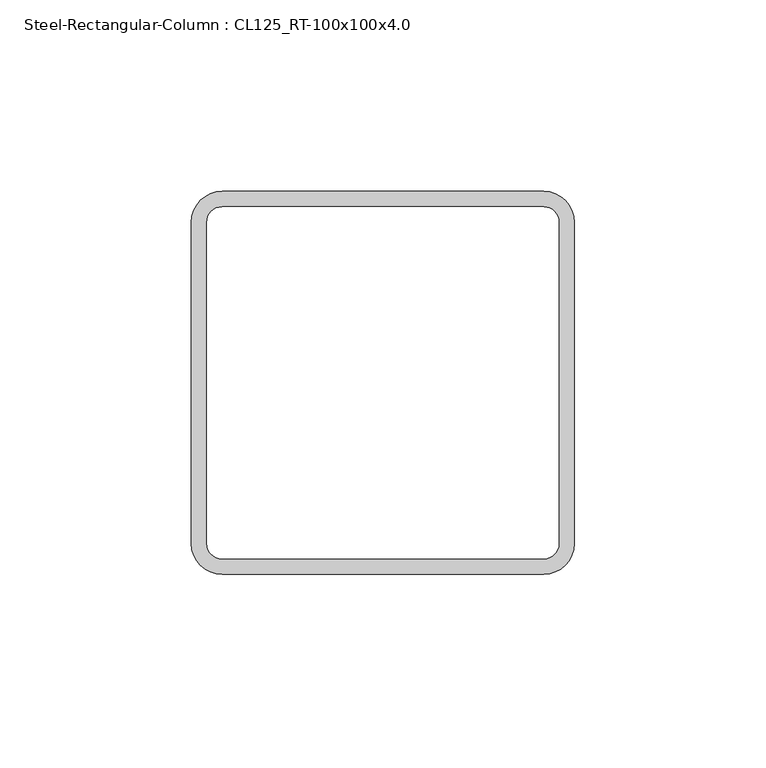
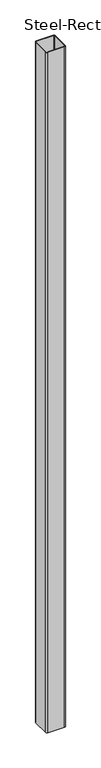
"""IFC4 building model written with IfcOpenShell, lengths in millimetres: column geometry, Steel-Rectangular-Column : CL125_RT-100x100x4.0."""

import ifcopenshell
import ifcopenshell.guid

model = None  # the IFC model being written
_history = None  # IfcOwnerHistory: only IFC2X3 demands one
_inside = {}  # id of a spatial element -> (the spatial element, [elements in it])
_under = {}  # id of a project, library or spatial element -> (it, [spatial elements below it])
_declared = {}  # id of a project -> (the project, [libraries it declares])
_typed = {}  # id of a type object -> (the type object, [elements of that type])
_made_of = {}  # id of a material, layer set ... -> (it, [elements and type objects made of it])


def new_model(schema):
    """Start an empty IFC model of exactly this schema.

    Asked for "IFC4X3", IfcOpenShell would pick the latest addendum, in which some entities
    have other attributes; the version numbers below select the first issue.
    IFC2X3 requires an IfcOwnerHistory on every rooted entity: one is made here for all.
    """
    global model, _history
    if schema == "IFC4X3":
        model = ifcopenshell.file(schema_version=(4, 3, 0, 0))
    else:
        model = ifcopenshell.file(schema=schema)
    _inside.clear()
    _under.clear()
    _declared.clear()
    _typed.clear()
    _made_of.clear()
    _history = None
    if model.schema == "IFC2X3":
        org = make("IfcOrganization", Name="unknown")
        user = make(
            "IfcPersonAndOrganization",
            ThePerson=make("IfcPerson", FamilyName="unknown"),
            TheOrganization=org,
        )
        app = make(
            "IfcApplication",
            ApplicationDeveloper=org,
            Version="unknown",
            ApplicationFullName="unknown",
            ApplicationIdentifier="unknown",
        )
        _history = make(
            "IfcOwnerHistory",
            OwningUser=user,
            OwningApplication=app,
            ChangeAction="ADDED",
            CreationDate=0,
        )
    return model


def make(cls, **values):
    """One entity of the class cls with the attributes given. An attribute that is None is left unset."""
    return model.create_entity(
        cls, **{name: value for name, value in values.items() if value is not None}
    )


def rooted(cls, **values):
    """An entity with a GlobalId (a new one), such as an element, a storey or a relation."""
    return make(cls, GlobalId=ifcopenshell.guid.new(), OwnerHistory=_history, **values)


def si_unit(unit_type, name, prefix=None):
    """IfcSIUnit, for example si_unit("LENGTHUNIT", "METRE", prefix="MILLI")."""
    return make("IfcSIUnit", UnitType=unit_type, Prefix=prefix, Name=name)


def assignment(units):
    """IfcUnitAssignment: the units of a project."""
    return None if units is None else make("IfcUnitAssignment", Units=units)


def point(xyz):
    """IfcCartesianPoint."""
    return None if xyz is None else make("IfcCartesianPoint", Coordinates=xyz)


def direction(xyz):
    """IfcDirection."""
    return None if xyz is None else make("IfcDirection", DirectionRatios=xyz)


def frame(location, z_axis=None, x_axis=None):
    """IfcAxis2Placement3D, a coordinate frame: its origin and axes. An axis left out is left unset."""
    return make(
        "IfcAxis2Placement3D",
        Location=point(location),
        Axis=direction(z_axis),
        RefDirection=direction(x_axis),
    )


def frame_2d(location, x_axis=None):
    """IfcAxis2Placement2D, a coordinate frame in the plane: its origin and x axis."""
    return make(
        "IfcAxis2Placement2D", Location=point(location), RefDirection=direction(x_axis)
    )


def origin():
    """The frame at (0, 0, 0) with its axes left unset."""
    return frame((0.0, 0.0, 0.0))


def place(relative_to, where):
    """IfcLocalPlacement: puts the frame where relative to a parent placement (None: the world)."""
    return make(
        "IfcLocalPlacement", PlacementRelTo=relative_to, RelativePlacement=where
    )


def context(
    kind, dimensions, precision=None, world=None, true_north=None, identifier=None
):
    """IfcGeometricRepresentationContext, for example the 3D "Model" context."""
    return make(
        "IfcGeometricRepresentationContext",
        ContextIdentifier=identifier,
        ContextType=kind,
        CoordinateSpaceDimension=dimensions,
        Precision=precision,
        WorldCoordinateSystem=world,
        TrueNorth=true_north,
    )


def project(units=None, contexts=None):
    """IfcProject with its units and contexts."""
    return rooted(
        "IfcProject",
        Name="project",
        RepresentationContexts=contexts,
        UnitsInContext=assignment(units),
    )


def spatial(cls, under=None, at=None, **own):
    """A site, building, storey or space (cls), placed at a placement, below another one or the project."""
    s = rooted(cls, ObjectPlacement=at, **own)
    if under is not None:
        _under.setdefault(under.id(), (under, []))[1].append(s)
    return s


def polyline(points):
    """IfcPolyline through the points."""
    return make("IfcPolyline", Points=[point(p) for p in points])


def circle_curve(where, radius):
    """IfcCircle in the frame where."""
    return make("IfcCircle", Position=where, Radius=radius)


def trimmed(basis, trim1, trim2, sense, master):
    """IfcTrimmedCurve: the piece of a basis curve between two trims."""
    return make(
        "IfcTrimmedCurve",
        BasisCurve=basis,
        Trim1=trim1,
        Trim2=trim2,
        SenseAgreement=sense,
        MasterRepresentation=master,
    )


def segment(curve, same_sense, transition):
    """IfcCompositeCurveSegment."""
    return make(
        "IfcCompositeCurveSegment",
        Transition=transition,
        SameSense=same_sense,
        ParentCurve=curve,
    )


def composite_curve(segments, self_intersect=None):
    """IfcCompositeCurve: segments joined end to end."""
    return make("IfcCompositeCurve", Segments=segments, SelfIntersect=self_intersect)


def outline(outer, holes=None, kind="AREA"):
    """IfcArbitraryClosedProfileDef: a profile drawn as a closed curve; with holes, ...WithVoids."""
    if holes is None:
        return make("IfcArbitraryClosedProfileDef", ProfileType=kind, OuterCurve=outer)
    return make(
        "IfcArbitraryProfileDefWithVoids",
        ProfileType=kind,
        OuterCurve=outer,
        InnerCurves=holes,
    )


def extrude(swept, where, along, depth):
    """IfcExtrudedAreaSolid: the profile swept, set in the frame where, extruded along a direction by depth."""
    return make(
        "IfcExtrudedAreaSolid",
        SweptArea=swept,
        Position=where,
        ExtrudedDirection=direction(along),
        Depth=depth,
    )


def shape(context_of_items, identifier, shape_type, items):
    """IfcShapeRepresentation: the items that make up one representation, for example the "Body"."""
    return make(
        "IfcShapeRepresentation",
        ContextOfItems=context_of_items,
        RepresentationIdentifier=identifier,
        RepresentationType=shape_type,
        Items=items,
    )


def source(mapping_origin, context_of_items, identifier, shape_type, items):
    """IfcRepresentationMap: a shape defined once, which mapped items show again and again."""
    return make(
        "IfcRepresentationMap",
        MappingOrigin=mapping_origin,
        MappedRepresentation=shape(context_of_items, identifier, shape_type, items),
    )


def transform(
    local_origin,
    x_axis=None,
    y_axis=None,
    z_axis=None,
    scale=None,
    scale2=None,
    scale3=None,
    uniform=True,
):
    """IfcCartesianTransformationOperator3D, or its non-uniform kind. x_axis, y_axis, z_axis: its Axis1, 2, 3."""
    if uniform:
        return make(
            "IfcCartesianTransformationOperator3D",
            Axis1=direction(x_axis),
            Axis2=direction(y_axis),
            LocalOrigin=point(local_origin),
            Scale=scale,
            Axis3=direction(z_axis),
        )
    return make(
        "IfcCartesianTransformationOperator3DnonUniform",
        Axis1=direction(x_axis),
        Axis2=direction(y_axis),
        LocalOrigin=point(local_origin),
        Scale=scale,
        Axis3=direction(z_axis),
        Scale2=scale2,
        Scale3=scale3,
    )


def mapped(mapping_source, mapping_target):
    """IfcMappedItem: shows the shape of a source again, moved by a transform."""
    return make(
        "IfcMappedItem", MappingSource=mapping_source, MappingTarget=mapping_target
    )


def made_of(thing, what):
    """Note that an element or type object is made of a material, layer set ...; save() writes the relation."""
    if what is not None:
        _made_of.setdefault(what.id(), (what, []))[1].append(thing)
    return thing


def element(
    cls,
    number,
    at=None,
    inside=None,
    cuts=None,
    type_object=None,
    material=None,
    context=None,
    identifier="Body",
    shape_type=None,
    held_by="IfcProductDefinitionShape",
    body=None,
    shapes=None,
    **own,
):
    """One element of the class cls, such as IfcWall. Its Tag is "e" and its number.

    at: its placement. inside: the storey or other place that contains it. cuts: it is an
    opening in that element (IfcRelVoidsElement). A single representation is given by context,
    identifier, shape_type and body (its items); several are given by shapes. held_by: the class
    of the entity that holds the representations. save() writes the other relations.
    """
    e = rooted(cls, Tag="e%d" % number, ObjectPlacement=at, **own)
    if body is not None:
        shapes = [shape(context, identifier, shape_type, body)]
    if shapes is not None:
        e.Representation = make(held_by, Representations=shapes)
    if inside is not None:
        _inside.setdefault(inside.id(), (inside, []))[1].append(e)
    if cuts is not None:
        rooted(
            "IfcRelVoidsElement", RelatingBuildingElement=cuts, RelatedOpeningElement=e
        )
    if type_object is not None:
        _typed.setdefault(type_object.id(), (type_object, []))[1].append(e)
    return made_of(e, material)


def aggregate(whole, parts):
    """IfcRelAggregates: a whole, such as a stair, and the parts it consists of."""
    return rooted("IfcRelAggregates", RelatingObject=whole, RelatedObjects=parts)


def save(model, path):
    """Write the relations noted so far, then the file.

    IfcRelAggregates (storeys below a building ...), IfcRelContainedInSpatialStructure (elements
    in a storey), IfcRelDefinesByType, IfcRelAssociatesMaterial and IfcRelDeclares: one each for
    every whole, place, type object, material and project.
    """
    for whole, parts in _under.values():
        aggregate(whole, parts)
    for where, things in _inside.values():
        rooted(
            "IfcRelContainedInSpatialStructure",
            RelatedElements=things,
            RelatingStructure=where,
        )
    for kind, things in _typed.values():
        rooted("IfcRelDefinesByType", RelatedObjects=things, RelatingType=kind)
    for what, things in _made_of.values():
        rooted("IfcRelAssociatesMaterial", RelatedObjects=things, RelatingMaterial=what)
    for by, libraries in _declared.values():
        rooted("IfcRelDeclares", RelatingContext=by, RelatedDefinitions=libraries)
    model.write(path)


def steel_rectangular_column_cl125_rt_100x100x4_0_aaa137b4(model_context):
    return source(origin(), model_context, "Body", "SweptSolid", [
        extrude(outline(composite_curve([segment(trimmed(circle_curve(frame_2d((42.0, 42.0)), 8.0), [point((42.0, 50.0))], [point((50.0, 42.0))], False, "CARTESIAN"), True, "CONTINUOUS"), segment(polyline([(50.0, 42.0), (50.0, -42.0)]), True, "CONTINUOUS"), segment(trimmed(circle_curve(frame_2d((42.0, -42.0)), 8.0), [point((50.0, -42.0))], [point((42.0, -50.0))], False, "CARTESIAN"), True, "CONTINUOUS"), segment(polyline([(42.0, -50.0), (-42.0, -50.0)]), True, "CONTINUOUS"), segment(trimmed(circle_curve(frame_2d((-42.0, -42.0)), 8.0), [point((-42.0, -50.0))], [point((-50.0, -42.0))], False, "CARTESIAN"), True, "CONTINUOUS"), segment(polyline([(-50.0, -42.0), (-50.0, 42.0)]), True, "CONTINUOUS"), segment(trimmed(circle_curve(frame_2d((-42.0, 42.0)), 8.0), [point((-50.0, 42.0))], [point((-42.0, 50.0))], False, "CARTESIAN"), True, "CONTINUOUS"), segment(polyline([(-42.0, 50.0), (42.0, 50.0)]), True, "CONTINUOUS")], self_intersect=False), holes=[composite_curve([segment(polyline([(42.0, 46.0), (-42.0, 46.0)]), True, "CONTINUOUS"), segment(trimmed(circle_curve(frame_2d((-42.0, 42.0)), 4.0), [point((-42.0, 46.0))], [point((-46.0, 42.0))], True, "CARTESIAN"), True, "CONTINUOUS"), segment(polyline([(-46.0, 42.0), (-46.0, -42.0)]), True, "CONTINUOUS"), segment(trimmed(circle_curve(frame_2d((-42.0, -42.0)), 4.0), [point((-46.0, -42.0))], [point((-42.0, -46.0))], True, "CARTESIAN"), True, "CONTINUOUS"), segment(polyline([(-42.0, -46.0), (42.0, -46.0)]), True, "CONTINUOUS"), segment(trimmed(circle_curve(frame_2d((42.0, -42.0)), 4.0), [point((42.0, -46.0))], [point((46.0, -42.0))], True, "CARTESIAN"), True, "CONTINUOUS"), segment(polyline([(46.0, -42.0), (46.0, 42.0)]), True, "CONTINUOUS"), segment(trimmed(circle_curve(frame_2d((42.0, 42.0)), 4.0), [point((46.0, 42.0))], [point((42.0, 46.0))], True, "CARTESIAN"), True, "CONTINUOUS")], self_intersect=False)]), frame((0.0, 0.0, 1400.0), z_axis=(0.0, 0.0, 1.0), x_axis=(1.0, 0.0, 0.0)), (0.0, 0.0, 1.0), 3600.0),
    ])


if __name__ == "__main__":
    model = new_model("IFC4")
    model_context = context("Model", 3, world=origin())
    ifc_project = project(units=[si_unit("LENGTHUNIT", "METRE", prefix="MILLI")], contexts=[model_context])
    site = spatial("IfcSite", under=ifc_project)
    building = spatial("IfcBuilding", under=site)
    placement = place(None, origin())
    steel_rectangular_column_cl125_rt_100x100x4_0_shape = steel_rectangular_column_cl125_rt_100x100x4_0_aaa137b4(model_context)
    element("IfcColumn", 1, ObjectType="Steel-Rectangular-Column : CL125_RT-100x100x4.0", at=placement, inside=building, context=model_context, shape_type="MappedRepresentation", body=[
        mapped(steel_rectangular_column_cl125_rt_100x100x4_0_shape, transform((0.0, 0.0, 0.0), x_axis=(1.0, 0.0, 0.0), y_axis=(0.0, 1.0, 0.0), z_axis=(0.0, 0.0, 1.0))),
    ])
    save(model, "model.ifc")

# Revit data of these elements
# Type "Steel-Rectangular-Column : CL125_RT-100x100x4.0"
#   Surface Area = 0.386 m²/m
#   b = 100 mm
#   h = 100 mm
#   tr = 8 mm
#   t = 4 mm
#   Section Area = 14.95 cm²
#   Mass per Unit Length = 11.70 kg/m
#   hec_material4 [instance default] = none
#   hec_material3 [instance default] = none
#   hec_material2 [instance default] = none
#   hec_material1 [instance default] = none
#   Structural Material [instance default] = Steel, 45-345
# Element 1 (IfcColumn, "Steel-Rectangular-Column : CL125_RT-100x100x4.0")
#   Structural Material = S01AA007-00001_Main Steel Structure Fabrication Work_Shelter/Building_Girth & Purlin
#   Materials on its faces: "S01AA007-00001_Main Steel Structure Fabrication Work_Shelter/Building_Girth & Purlin"
# Materials
#   "Steel, 45-345": class "Metal", colour RGB 189 187 185, transparency 0, Description = "Steel 345 MPa", Cost = 0
#   "S01AA007-00001_Main Steel Structure Fabrication Work_Shelter/Building_Girth & Purlin": class "Metal", colour RGB 120 120 120, transparency 0, Comments = "(30KG/M>Weight)", Description = "Structural steel 50ksi", W00) Work Master Code = "S01AA007-00001", W01) Work Master_Lv1 = "Main Steel Structure Fabrication Work", W02) Work Master_Lv2 = "Shelter/Building", W03) Work Master_Spec.1 = "Girth & Purlin", Cost = 0
